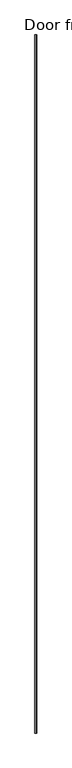
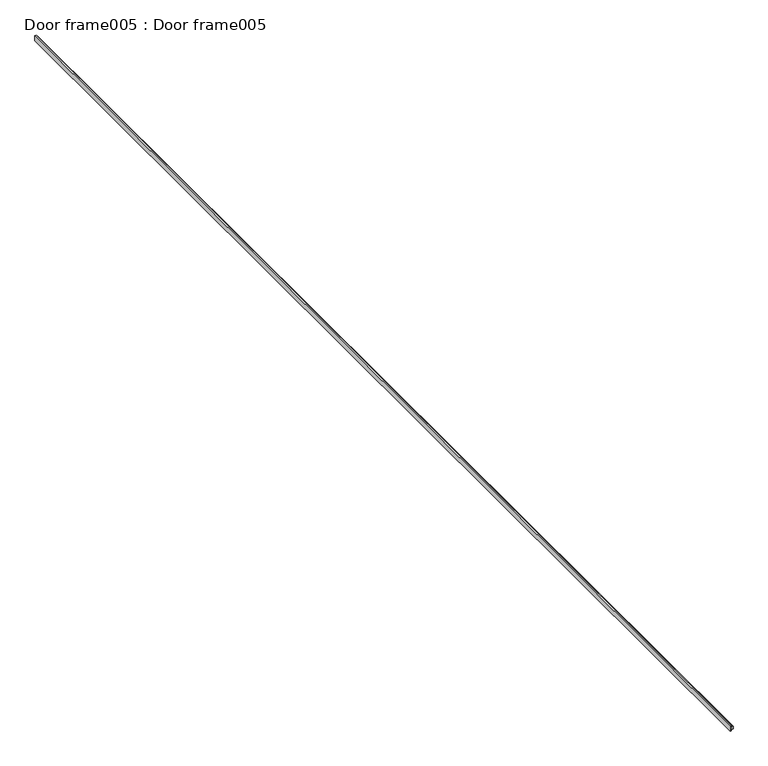
"""IFC4 building model written with IfcOpenShell, lengths in millimetres: proxy geometry, Door frame005 : Door frame005."""

from ifc_helpers import new_model, si_unit, frame, origin, place, context, project, spatial, polyline, outline, extrude, source, transform, mapped, element, save


def door_frame005_door_frame005_abb10e86(model_context):
    return source(origin(), model_context, "Body", "SweptSolid", [
        extrude(outline(polyline([(36678.7014343, 15555.3292246), (36678.7014343, 15557.5465976), (36682.2000947, 15557.5465976), (36682.2000947, 15559.3245976), (36680.8030947, 15559.3245976), (36680.8030947, 15560.3913976), (36685.3750947, 15560.3913976), (36685.3750947, 15559.3245976), (36683.9780947, 15559.3245976), (36683.9780947, 15557.546547), (36687.4772673, 15557.546547), (36687.4772673, 15555.3292246), (36678.7014343, 15555.3292246)])), frame((0.0, -1052.8906567, 0.0), z_axis=(0.0, 1.0, 0.0), x_axis=(0.0, 0.0, 1.0)), (0.0, 0.0, 1.0), 1999.85),
    ])


if __name__ == "__main__":
    model = new_model("IFC4")
    model_context = context("Model", 3, world=origin())
    ifc_project = project(units=[si_unit("LENGTHUNIT", "METRE", prefix="MILLI")], contexts=[model_context])
    site = spatial("IfcSite", under=ifc_project)
    building = spatial("IfcBuilding", under=site)
    placement = place(None, origin())
    door_frame005_door_frame005_shape = door_frame005_door_frame005_abb10e86(model_context)
    element("IfcBuildingElementProxy", 1, Name="Door frame005 : Door frame005", ObjectType="Door frame005 : Door frame005", at=placement, inside=building, context=model_context, shape_type="MappedRepresentation", body=[
        mapped(door_frame005_door_frame005_shape, transform((0.0, 0.0, 0.0), x_axis=(1.0, 0.0, 0.0), y_axis=(0.0, 1.0, 0.0), z_axis=(0.0, 0.0, 1.0))),
    ])
    save(model, "model.ifc")

# Revit data of these elements
# Type "Door frame005 : Door frame005"
#   NameOverride = "Door frame005"
# Element 1 (IfcBuildingElementProxy, "Door frame005 : Door frame005")
#   Materials on its faces: "FLEETWOOD SERIES T-3200 SINGLE SWING DOOR FRAME"
# Materials
#   "FLEETWOOD SERIES T-3200 SINGLE SWING DOOR FRAME": class "Unassigned", colour RGB 128 128 128, transparency 0, Cost = 0
